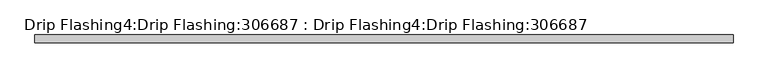
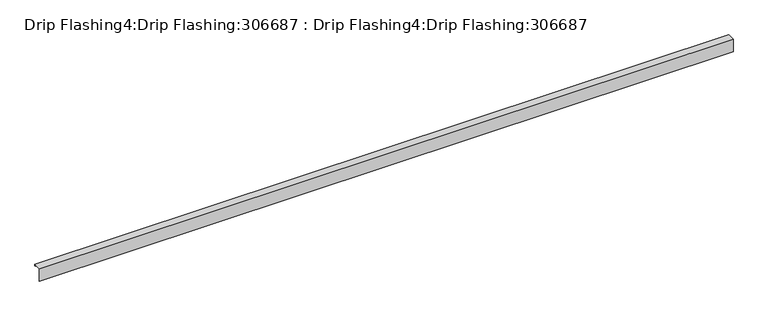
"""IFC4 building model written with IfcOpenShell, lengths in millimetres: proxy geometry, Drip Flashing4:Drip Flashing:306687 : Drip Flashing4:Drip Flashing:306687."""

from ifc_helpers import new_model, si_unit, frame, origin, place, context, project, spatial, polyline, outline, extrude, source, transform, mapped, element, save


def drip_flashing4_drip_flashing_306687_drip_flashing4_drip_12db65b6(model_context):
    return source(origin(), model_context, "Body", "SweptSolid", [
        extrude(outline(polyline([(10045.7124956, 37596.6323437), (10026.0274956, 37596.6323437), (10026.0274956, 37559.8023437), (10024.7574956, 37559.8023437), (10024.7574956, 37597.9023437), (10046.9824956, 37597.9023437), (10046.9824956, 37593.1525437), (10043.9800392, 37593.1525437), (10043.9800392, 37594.4225437), (10045.7124956, 37594.4225437), (10045.7124956, 37596.6323437)])), frame((-4455.0628198, 0.0, 0.0), z_axis=(1.0, 0.0, 0.0), x_axis=(0.0, 1.0, 0.0)), (0.0, 0.0, 1.0), 1999.85),
    ])


if __name__ == "__main__":
    model = new_model("IFC4")
    model_context = context("Model", 3, world=origin())
    ifc_project = project(units=[si_unit("LENGTHUNIT", "METRE", prefix="MILLI")], contexts=[model_context])
    site = spatial("IfcSite", under=ifc_project)
    building = spatial("IfcBuilding", under=site)
    placement = place(None, origin())
    drip_flashing4_drip_flashing_306687_drip_flashing4_drip_shape = drip_flashing4_drip_flashing_306687_drip_flashing4_drip_12db65b6(model_context)
    element("IfcBuildingElementProxy", 1, Name="Drip Flashing4:Drip Flashing:306687 : Drip Flashing4:Drip Flashing:306687", ObjectType="Drip Flashing4:Drip Flashing:306687 : Drip Flashing4:Drip Flashing:306687", at=placement, inside=building, context=model_context, shape_type="MappedRepresentation", body=[
        mapped(drip_flashing4_drip_flashing_306687_drip_flashing4_drip_shape, transform((0.0, 0.0, 0.0), x_axis=(1.0, 0.0, 0.0), y_axis=(0.0, 1.0, 0.0), z_axis=(0.0, 0.0, 1.0))),
    ])
    save(model, "model.ifc")

# Revit data of these elements
# Type "Drip Flashing4:Drip Flashing:306687 : Drip Flashing4:Drip Flashing:306687"
#   NameOverride = "Drip Flashing4:Drip Flashing:306687"
#   ObjectTypeOverride = "Drip Flashing4:Drip Flashing"
#   Reference = "Drip Flashing"
#   Category = "Generic Models"
#   Tag = "306687"
# Element 1 (IfcBuildingElementProxy, "Drip Flashing4:Drip Flashing:306687 : Drip Flashing4:Drip Flashing:306687")
#   Materials on its faces: "COPPER STUCCO J BEAD"
# Materials
#   "COPPER STUCCO J BEAD": class "Unassigned", colour RGB 251 232 155, transparency 0, Cost = 0
